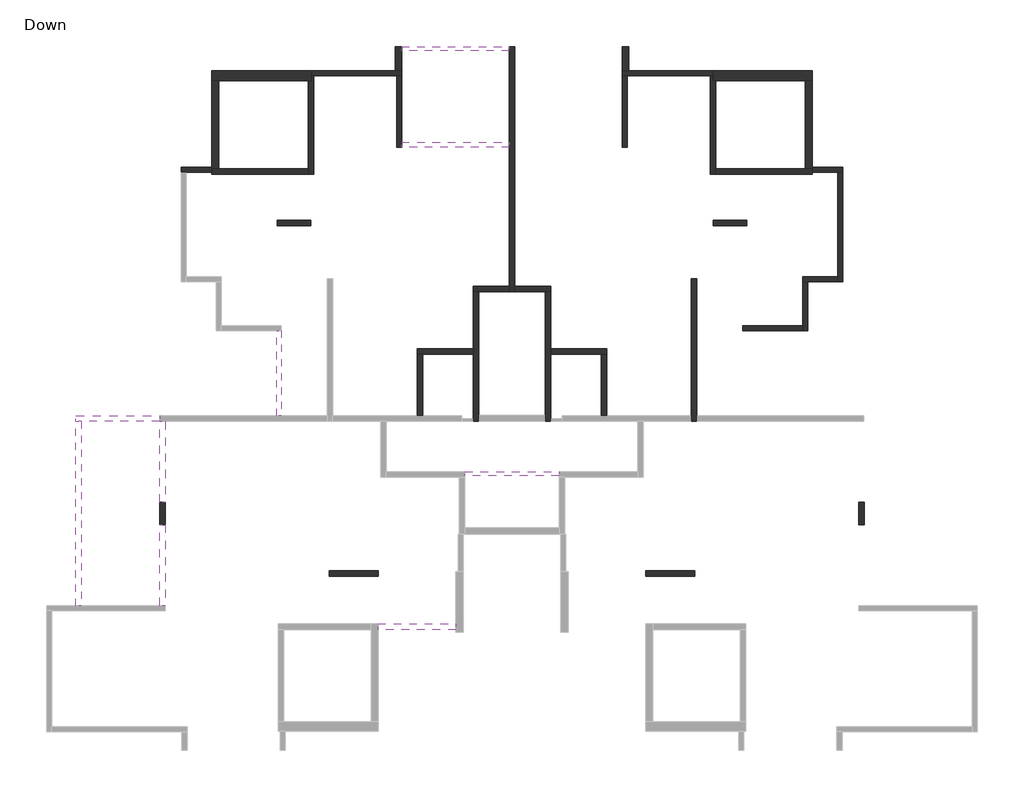
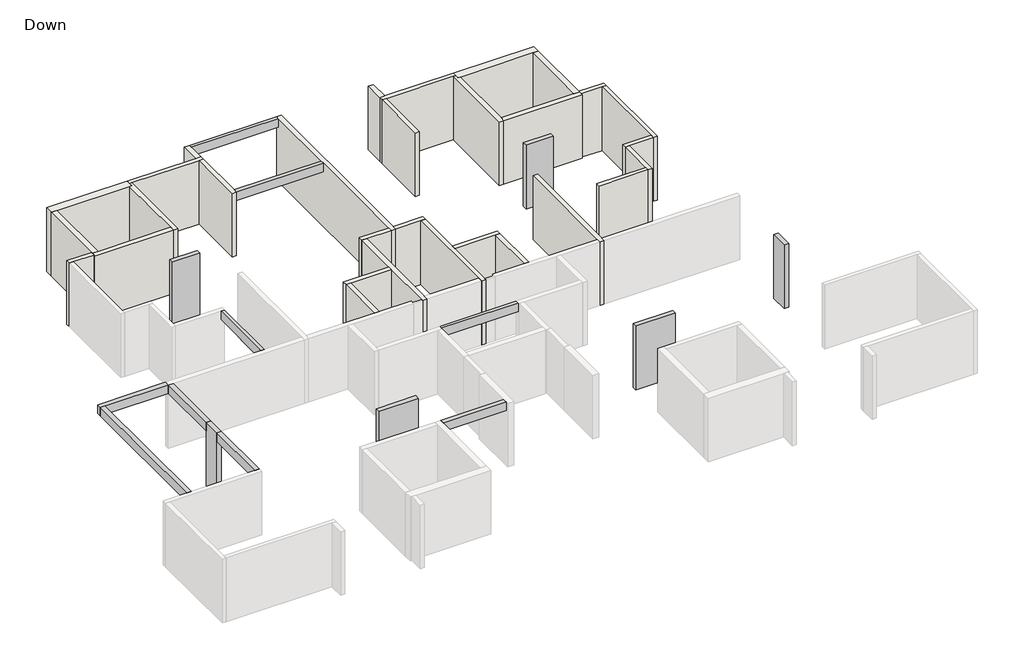
# One storey, part 2 of 2: 30 walls, 9 beams, 6 columns.
"""IFC4 building model written with IfcOpenShell, lengths in millimetres."""

from ifc_helpers import new_model, si_unit, origin, origin_with_axes, place, context, project, spatial, polyline, outline, extrude, faceted_brep, element, save

model = new_model("IFC4")

# Units and contexts
model_context = context("Model", 3, world=origin())
ifc_project = project(units=[si_unit("LENGTHUNIT", "METRE", prefix="MILLI")], contexts=[model_context])

# Site, building, storey
site = spatial("IfcSite", under=ifc_project)
building = spatial("IfcBuilding", under=site)
storey = spatial("IfcBuildingStorey", under=building, Name="Down", Elevation=0.0)

# Beams
placement = place(None, origin())
element("IfcBeam", 1, ObjectType="Concrete Rectengular Beam : 15/40", at=placement, inside=storey, context=model_context, shape_type="Brep", body=[
    faceted_brep([(-7447.2504016, 3105.4959573, 2970.0), (-7597.2504016, 3105.4959573, 2970.0), (-7597.2504016, 53.6346435, 2970.0), (-7447.2504016, 53.6346435, 2970.0), (-7597.2504016, 3105.4959573, 2570.0), (-7597.2504016, 53.6346435, 2570.0), (-7447.2504016, 3105.4959573, 2570.0), (-7447.2504016, 53.6346435, 2570.0), (-7447.2504016, 53.6346435, 2760.0), (-7447.2504016, 3105.4959573, 2760.0)], [[[0, 1, 2, 3]], [[1, 4, 5, 2]], [[4, 6, 7, 5]], [[0, 3, 8, 7, 6, 9]], [[1, 0, 9, 6, 4]], [[3, 2, 5, 7, 8]]]),
])
element("IfcBeam", 2, ObjectType="Concrete Rectengular Beam : 15/40", at=placement, inside=storey, context=model_context, shape_type="Brep", body=[
    faceted_brep([(-3124.7686498, 13277.6127456, 2970.0), (-3124.7686498, 13127.6127456, 2970.0), (722.5306203, 13127.6127456, 2970.0), (722.5306203, 13277.6127456, 2970.0), (-3124.7686498, 13127.6127456, 2760.0), (-3124.7686498, 13127.6127456, 2570.0), (722.5306203, 13127.6127456, 2570.0), (722.5306203, 13127.6127456, 2760.0), (-3124.7686498, 13277.6127456, 2570.0), (722.5306203, 13277.6127456, 2570.0)], [[[0, 1, 2, 3]], [[1, 4, 5, 6, 7, 2]], [[5, 8, 9, 6]], [[8, 0, 3, 9]], [[1, 0, 8, 5, 4]], [[3, 2, 7, 6, 9]]]),
])
element("IfcBeam", 3, ObjectType="Concrete Rectengular Beam : 15/40", at=placement, inside=storey, context=model_context, shape_type="Brep", body=[
    faceted_brep([(-874.5073169, -1946.3653565, 2970.0), (-874.5073169, -2096.3653565, 2970.0), (2519.5685574, -2096.3653565, 2970.0), (2519.5685574, -1946.3653565, 2970.0), (-874.5073169, -2096.3653565, 2760.0), (-874.5073169, -2096.3653565, 2570.0), (2519.5685574, -2096.3653565, 2570.0), (2519.5685574, -2096.3653565, 2760.0), (-874.5073169, -1946.3653565, 2570.0), (2519.5685574, -1946.3653565, 2570.0)], [[[0, 1, 2, 3]], [[1, 4, 5, 6, 7, 2]], [[5, 8, 9, 6]], [[8, 0, 3, 9]], [[1, 0, 8, 5, 4]], [[3, 2, 7, 6, 9]]]),
])
element("IfcBeam", 4, ObjectType="Concrete Rectengular Beam : 18/40", at=placement, inside=storey, context=model_context, shape_type="Brep", body=[
    faceted_brep([(-3124.7686498, 9859.0725997, 2970.0), (-3124.7686498, 9679.0725997, 2970.0), (722.5306203, 9679.0725997, 2970.0), (722.5306203, 9859.0725997, 2970.0), (-3124.7686498, 9679.0725997, 2760.0), (-3124.7686498, 9679.0725997, 2570.0), (722.5306203, 9679.0725997, 2570.0), (722.5306203, 9679.0725997, 2760.0), (-3124.7686498, 9859.0725997, 2570.0), (722.5306203, 9859.0725997, 2570.0), (-3124.7686498, 9859.0725997, 2760.0), (722.5306203, 9859.0725997, 2760.0)], [[[0, 1, 2, 3]], [[2, 1, 4, 5, 6, 7]], [[5, 8, 9, 6]], [[8, 10, 0, 3, 11, 9]], [[1, 0, 10, 8, 5, 4]], [[3, 2, 7, 6, 9, 11]]]),
])
element("IfcBeam", 5, ObjectType="Concrete Rectengular Beam : 20/40", at=placement, inside=storey, context=model_context, shape_type="Brep", body=[
    faceted_brep([(-14797.7613505, 53.6346435, 2970.0), (-14797.7613505, -146.3653565, 2970.0), (-14597.7613505, -146.3653565, 2970.0), (-11795.1336133, -146.3653565, 2970.0), (-11795.1336133, 53.6346435, 2970.0), (-14797.7613505, 53.6346435, 2570.0), (-11795.1336133, 53.6346435, 2570.0), (-14797.7613505, -146.3653565, 2570.0), (-11795.1336133, -146.3653565, 2570.0), (-14597.7613505, -146.3653565, 2570.0), (-11795.1336133, -146.3653565, 2760.0)], [[[0, 1, 2, 3, 4]], [[5, 0, 4, 6]], [[7, 5, 6, 8, 9]], [[1, 7, 9, 8, 10, 3, 2]], [[1, 0, 5, 7]], [[4, 3, 10, 8, 6]]]),
])
element("IfcBeam", 6, ObjectType="Concrete Rectengular Beam : 20/40", at=placement, inside=storey, context=model_context, shape_type="Brep", body=[
    faceted_brep([(-14797.7613505, -6750.8420555, 2970.0), (-14597.7613505, -6750.8420555, 2970.0), (-14597.7613505, -146.3653565, 2970.0), (-14797.7613505, -146.3653565, 2970.0), (-14797.7613505, -6750.8420555, 2570.0), (-14797.7613505, -146.3653565, 2570.0), (-14597.7613505, -6750.8420555, 2570.0), (-14597.7613505, -146.3653565, 2570.0), (-14597.7613505, -6750.8420555, 2760.0), (-14597.7613505, -146.3653565, 2760.0)], [[[0, 1, 2, 3]], [[4, 0, 3, 5]], [[6, 4, 5, 7]], [[1, 8, 6, 7, 9, 2]], [[1, 0, 4, 6, 8]], [[3, 2, 9, 7, 5]]]),
])
element("IfcBeam", 7, ObjectType="Concrete Rectengular Beam : 20/40", at=placement, inside=storey, context=model_context, shape_type="Brep", body=[
    faceted_brep([(-11795.1336133, -3042.8252106, 2970.0), (-11595.1336133, -3042.8252106, 2970.0), (-11595.1336133, -146.3653565, 2970.0), (-11795.1336133, -146.3653565, 2970.0), (-11795.1336133, -3042.8252106, 2570.0), (-11795.1336133, -146.3653565, 2760.0), (-11795.1336133, -146.3653565, 2570.0), (-11595.1336133, -3042.8252106, 2570.0), (-11595.1336133, -146.3653565, 2570.0), (-11595.1336133, -3042.8252106, 2760.0), (-11595.1336133, -146.3653565, 2760.0)], [[[0, 1, 2, 3]], [[4, 0, 3, 5, 6]], [[7, 4, 6, 8]], [[2, 1, 9, 7, 8, 10]], [[1, 0, 4, 7, 9]], [[3, 2, 10, 8, 6, 5]]]),
])
element("IfcBeam", 8, ObjectType="Concrete Rectengular Beam : 20/40", at=placement, inside=storey, context=model_context, shape_type="Brep", body=[
    faceted_brep([(-11595.1336133, -3842.8252106, 2970.0), (-11795.1336133, -3842.8252106, 2970.0), (-11795.1336133, -6750.8420555, 2970.0), (-11595.1336133, -6750.8420555, 2970.0), (-11795.1336133, -3842.8252106, 2570.0), (-11795.1336133, -6750.8420555, 2570.0), (-11795.1336133, -6750.8420555, 2760.0), (-11595.1336133, -3842.8252106, 2570.0), (-11595.1336133, -6750.8420555, 2570.0), (-11595.1336133, -6750.8420555, 2760.0), (-11595.1336133, -3842.8252106, 2760.0)], [[[0, 1, 2, 3]], [[1, 4, 5, 6, 2]], [[4, 7, 8, 5]], [[0, 3, 9, 8, 7, 10]], [[1, 0, 10, 7, 4]], [[3, 2, 6, 5, 8, 9]]]),
])
element("IfcBeam", 9, ObjectType="Concrete Rectengular Beam : 20/40", at=placement, inside=storey, context=model_context, shape_type="Brep", body=[
    faceted_brep([(-3973.7230475, -7395.8420555, 2970.0), (-3973.7230475, -7595.8420555, 2970.0), (-1189.5073169, -7595.8420555, 2970.0), (-1189.5073169, -7395.8420555, 2970.0), (-3973.7230475, -7595.8420555, 2570.0), (-1189.5073169, -7595.8420555, 2570.0), (-3973.7230475, -7395.8420555, 2570.0), (-1189.5073169, -7395.8420555, 2570.0), (-1189.5073169, -7395.8420555, 2760.0), (-3973.7230475, -7395.8420555, 2760.0)], [[[0, 1, 2, 3]], [[1, 4, 5, 2]], [[4, 6, 7, 5]], [[0, 3, 8, 7, 6, 9]], [[1, 0, 9, 6, 4]], [[3, 2, 5, 7, 8]]]),
])

# Columns
element("IfcColumn", 10, ObjectType="Concrete Rectengular Column : 20/120", at=placement, inside=storey, context=model_context, shape_type="Brep", body=[
    faceted_brep([(-7578.4912775, 7053.4886581, 0.0), (-6378.4912775, 7053.4886581, 0.0), (-6378.4912775, 6853.4886581, 0.0), (-7578.4912775, 6853.4886581, 0.0), (-7578.4912775, 7053.4886581, 2970.0), (-6378.4912775, 7053.4886581, 2970.0), (-6378.4912775, 7053.4886581, 2760.0), (-7578.4912775, 7053.4886581, 2760.0), (-6378.4912775, 6853.4886581, 2970.0), (-6378.4912775, 6853.4886581, 2760.0), (-7578.4912775, 6853.4886581, 2970.0), (-7578.4912775, 6853.4886581, 2760.0)], [[[0, 1, 2, 3]], [[4, 5, 6, 1, 0, 7]], [[5, 8, 9, 2, 1, 6]], [[8, 10, 11, 3, 2, 9]], [[10, 4, 7, 0, 3, 11]], [[4, 10, 8, 5]]]),
])
element("IfcColumn", 11, ObjectType="Concrete Rectengular Column : 20/120", at=placement, inside=storey, context=model_context, shape_type="Brep", body=[
    faceted_brep([(9223.5525181, 7053.4886581, 0.0), (9223.5525181, 6853.4886581, 0.0), (8023.5525181, 6853.4886581, 0.0), (8023.5525181, 7053.4886581, 0.0), (9223.5525181, 7053.4886581, 2970.0), (9223.5525181, 7053.4886581, 2760.0), (8023.5525181, 7053.4886581, 2760.0), (8023.5525181, 7053.4886581, 2970.0), (8023.5525181, 6853.4886581, 2760.0), (8023.5525181, 6853.4886581, 2970.0), (9223.5525181, 6853.4886581, 2760.0), (9223.5525181, 6853.4886581, 2970.0)], [[[0, 1, 2, 3]], [[4, 5, 0, 3, 6, 7]], [[7, 6, 3, 2, 8, 9]], [[9, 8, 2, 1, 10, 11]], [[11, 10, 1, 0, 5, 4]], [[4, 7, 9, 11]]]),
])
element("IfcColumn", 12, ObjectType="Concrete Rectengular Column : 20/175", at=placement, inside=storey, context=model_context, shape_type="Brep", body=[
    faceted_brep([(-5724.5402832, -5492.9594837, 0.0), (-3974.5402832, -5492.9594837, 0.0), (-3974.5402832, -5692.9594837, 0.0), (-5724.5402832, -5692.9594837, 0.0), (-5724.5402832, -5492.9594837, 2970.0), (-3974.5402832, -5492.9594837, 2970.0), (-3974.5402832, -5492.9594837, 2760.0), (-5724.5402832, -5492.9594837, 2760.0), (-3974.5402832, -5692.9594837, 2970.0), (-3974.5402832, -5692.9594837, 2760.0), (-5724.5402832, -5692.9594837, 2970.0), (-5724.5402832, -5692.9594837, 2760.0)], [[[0, 1, 2, 3]], [[4, 5, 6, 1, 0, 7]], [[5, 8, 9, 2, 1, 6]], [[8, 10, 11, 3, 2, 9]], [[10, 4, 7, 0, 3, 11]], [[4, 10, 8, 5]]]),
])
element("IfcColumn", 13, ObjectType="Concrete Rectengular Column : 20/175", at=placement, inside=storey, context=model_context, shape_type="Brep", body=[
    faceted_brep([(7369.6015237, -5492.9594837, 0.0), (7369.6015237, -5692.9594837, 0.0), (5619.6015237, -5692.9594837, 0.0), (5619.6015237, -5492.9594837, 0.0), (7369.6015237, -5492.9594837, 2970.0), (7369.6015237, -5492.9594837, 2760.0), (5619.6015237, -5492.9594837, 2760.0), (5619.6015237, -5492.9594837, 2970.0), (5619.6015237, -5692.9594837, 2760.0), (5619.6015237, -5692.9594837, 2970.0), (7369.6015237, -5692.9594837, 2760.0), (7369.6015237, -5692.9594837, 2970.0)], [[[0, 1, 2, 3]], [[4, 5, 0, 3, 6, 7]], [[7, 6, 3, 2, 8, 9]], [[9, 8, 2, 1, 10, 11]], [[11, 10, 1, 0, 5, 4]], [[4, 7, 9, 11]]]),
])
element("IfcColumn", 14, ObjectType="Concrete Rectengular Column : 20/80", at=placement, inside=storey, context=model_context, shape_type="SweptSolid", body=[
    extrude(outline(polyline([(-11595.1336133, -3042.8252106), (-11595.1336133, -3842.8252106), (-11795.1336133, -3842.8252106), (-11795.1336133, -3042.8252106), (-11595.1336133, -3042.8252106)])), origin_with_axes(), (0.0, 0.0, 1.0), 2970.0),
])
element("IfcColumn", 15, ObjectType="Concrete Rectengular Column : 20/80", at=placement, inside=storey, context=model_context, shape_type="SweptSolid", body=[
    extrude(outline(polyline([(13240.1948538, -3042.8252106), (13440.1948538, -3042.8252106), (13440.1948538, -3842.8252106), (13240.1948538, -3842.8252106), (13240.1948538, -3042.8252106)])), origin_with_axes(), (0.0, 0.0, 1.0), 2970.0),
])

# Walls
element("IfcWall", 16, ObjectType="18", at=placement, inside=storey, context=model_context, shape_type="Brep", body=[
    faceted_brep([(-6373.126314, 12225.4959573, 0.0), (-6273.126314, 12225.4959573, 0.0), (-3304.7686498, 12225.4959573, 0.0), (-3124.7686498, 12225.4959573, 0.0), (-3124.7686498, 12225.4959573, 2970.0), (-3304.7686498, 12225.4959573, 2970.0), (-6273.126314, 12225.4959573, 2970.0), (-6373.126314, 12225.4959573, 2970.0), (-6373.126314, 12405.4959573, 0.0), (-6373.126314, 12405.4959573, 2970.0), (-3354.7686498, 12405.4959573, 2970.0), (-3124.7686498, 12405.4959573, 2970.0), (-3124.7686498, 12405.4959573, 0.0), (-3354.7686498, 12405.4959573, 0.0)], [[[0, 1, 2, 3, 4, 5, 6, 7]], [[8, 9, 10, 11, 12, 13]], [[3, 2, 1, 0, 8, 13, 12]], [[7, 6, 5, 4, 11, 10, 9]], [[0, 7, 9, 8]], [[4, 3, 12, 11]]]),
])
element("IfcWall", 17, ObjectType="18", at=placement, inside=storey, context=model_context, shape_type="Brep", body=[
    faceted_brep([(-3304.7686498, 12225.4959573, 0.0), (-3304.7686498, 9679.0725997, 0.0), (-3304.7686498, 9679.0725997, 2760.0), (-3304.7686498, 9679.0725997, 2970.0), (-3304.7686498, 12225.4959573, 2970.0), (-3304.7686498, 12225.4959573, 2760.0), (-3124.7686498, 12225.4959573, 0.0), (-3124.7686498, 12225.4959573, 2970.0), (-3124.7686498, 9859.0725997, 2970.0), (-3124.7686498, 9679.0725997, 2970.0), (-3124.7686498, 9679.0725997, 0.0)], [[[0, 1, 2, 3, 4, 5]], [[6, 7, 8, 9, 10]], [[1, 0, 6, 10]], [[3, 2, 1, 10, 9]], [[4, 3, 9, 8, 7]], [[0, 5, 4, 7, 6]]]),
])
element("IfcWall", 18, ObjectType="18", at=placement, inside=storey, context=model_context, shape_type="Brep", body=[
    faceted_brep([(-9928.126314, 8955.4959573, 0.0), (-11023.126314, 8955.4959573, 0.0), (-11023.126314, 8955.4959573, 2970.0), (-9928.126314, 8955.4959573, 2970.0), (-9928.126314, 8775.4959573, 0.0), (-9928.126314, 8775.4959573, 2760.0), (-9928.126314, 8775.4959573, 2970.0), (-10843.126314, 8775.4959573, 2970.0), (-11023.126314, 8775.4959573, 2970.0), (-11023.126314, 8775.4959573, 0.0), (-10843.126314, 8775.4959573, 0.0), (-9928.126314, 8905.4959573, 0.0), (-9928.126314, 8905.4959573, 2970.0)], [[[0, 1, 2, 3]], [[4, 5, 6, 7, 8, 9, 10]], [[1, 0, 11, 4, 10, 9]], [[3, 2, 8, 7, 6, 12]], [[0, 3, 12, 6, 5, 4, 11]], [[2, 1, 9, 8]]]),
])
element("IfcWall", 19, ObjectType="18", at=placement, inside=storey, context=model_context, shape_type="Brep", body=[
    faceted_brep([(8018.1875546, 12405.4959573, 0.0), (4999.8298903, 12405.4959573, 0.0), (4769.8298903, 12405.4959573, 0.0), (4769.8298903, 12405.4959573, 2970.0), (4999.8298903, 12405.4959573, 2970.0), (8018.1875546, 12405.4959573, 2970.0), (8018.1875546, 12225.4959573, 0.0), (8018.1875546, 12225.4959573, 2970.0), (7918.1875546, 12225.4959573, 2970.0), (4949.8298903, 12225.4959573, 2970.0), (4769.8298903, 12225.4959573, 2970.0), (4769.8298903, 12225.4959573, 0.0), (4949.8298903, 12225.4959573, 0.0), (7918.1875546, 12225.4959573, 0.0)], [[[0, 1, 2, 3, 4, 5]], [[6, 7, 8, 9, 10, 11, 12, 13]], [[2, 1, 0, 6, 13, 12, 11]], [[5, 4, 3, 10, 9, 8, 7]], [[0, 5, 7, 6]], [[3, 2, 11, 10]]]),
])
element("IfcWall", 20, ObjectType="18", at=placement, inside=storey, context=model_context, shape_type="Brep", body=[
    faceted_brep([(4769.8298903, 12225.4959573, 0.0), (4769.8298903, 9679.0725997, 0.0), (4769.8298903, 9679.0725997, 2570.0), (4769.8298903, 9679.0725997, 2970.0), (4769.8298903, 9859.0725997, 2970.0), (4769.8298903, 12225.4959573, 2970.0), (4949.8298903, 12225.4959573, 0.0), (4949.8298903, 12225.4959573, 2760.0), (4949.8298903, 12225.4959573, 2970.0), (4949.8298903, 9679.0725997, 2970.0), (4949.8298903, 9679.0725997, 2760.0), (4949.8298903, 9679.0725997, 0.0)], [[[0, 1, 2, 3, 4, 5]], [[6, 7, 8, 9, 10, 11]], [[1, 0, 6, 11]], [[3, 2, 1, 11, 10, 9]], [[5, 4, 3, 9, 8]], [[0, 5, 8, 7, 6]]]),
])
element("IfcWall", 21, ObjectType="18", at=placement, inside=storey, context=model_context, shape_type="Brep", body=[
    faceted_brep([(11573.1875546, 8775.4959573, 0.0), (12488.1875546, 8775.4959573, 0.0), (12668.1875546, 8775.4959573, 0.0), (12668.1875546, 8775.4959573, 2970.0), (12488.1875546, 8775.4959573, 2970.0), (11573.1875546, 8775.4959573, 2970.0), (11573.1875546, 8775.4959573, 2760.0), (11573.1875546, 8955.4959573, 0.0), (11573.1875546, 8955.4959573, 2970.0), (12668.1875546, 8955.4959573, 2970.0), (12668.1875546, 8955.4959573, 0.0), (11573.1875546, 8905.4959573, 0.0), (11573.1875546, 8905.4959573, 2970.0)], [[[0, 1, 2, 3, 4, 5, 6]], [[7, 8, 9, 10]], [[2, 1, 0, 11, 7, 10]], [[5, 4, 3, 9, 8, 12]], [[0, 6, 5, 12, 8, 7, 11]], [[3, 2, 10, 9]]]),
])
element("IfcWall", 22, ObjectType="18", at=placement, inside=storey, context=model_context, shape_type="Brep", body=[
    faceted_brep([(12488.1875546, 8775.4959573, 0.0), (12488.1875546, 5035.4959573, 0.0), (12488.1875546, 4855.4959573, 0.0), (12488.1875546, 4855.4959573, 2970.0), (12488.1875546, 5035.4959573, 2970.0), (12488.1875546, 8775.4959573, 2970.0), (12488.1875546, 8775.4959573, 2760.0), (12668.1875546, 8775.4959573, 0.0), (12668.1875546, 8775.4959573, 2970.0), (12668.1875546, 4855.4959573, 2970.0), (12668.1875546, 4855.4959573, 0.0)], [[[0, 1, 2, 3, 4, 5, 6]], [[7, 8, 9, 10]], [[2, 1, 0, 7, 10]], [[5, 4, 3, 9, 8]], [[0, 6, 5, 8, 7]], [[3, 2, 10, 9]]]),
])
element("IfcWall", 23, ObjectType="18", at=placement, inside=storey, context=model_context, shape_type="Brep", body=[
    faceted_brep([(12488.1875546, 5035.4959573, 0.0), (11240.6852706, 5035.4959573, 0.0), (11240.6852706, 5035.4959573, 2760.0), (11240.6852706, 5035.4959573, 2970.0), (12488.1875546, 5035.4959573, 2970.0), (12488.1875546, 5035.4959573, 2760.0), (12488.1875546, 4855.4959573, 0.0), (12488.1875546, 4855.4959573, 2970.0), (11420.6852706, 4855.4959573, 2970.0), (11240.6852706, 4855.4959573, 2970.0), (11240.6852706, 4855.4959573, 0.0), (11420.6852706, 4855.4959573, 0.0)], [[[0, 1, 2, 3, 4, 5]], [[6, 7, 8, 9, 10, 11]], [[1, 0, 6, 11, 10]], [[4, 3, 9, 8, 7]], [[0, 5, 4, 7, 6]], [[3, 2, 1, 10, 9]]]),
])
element("IfcWall", 24, ObjectType="18", at=placement, inside=storey, context=model_context, shape_type="Brep", body=[
    faceted_brep([(11240.6852706, 4855.4959573, 0.0), (11240.6852706, 3285.4959573, 0.0), (11240.6852706, 3105.4959573, 0.0), (11240.6852706, 3105.4959573, 2970.0), (11240.6852706, 3285.4959573, 2970.0), (11240.6852706, 4855.4959573, 2970.0), (11420.6852706, 4855.4959573, 0.0), (11420.6852706, 4855.4959573, 2970.0), (11420.6852706, 3105.4959573, 2970.0), (11420.6852706, 3105.4959573, 0.0)], [[[0, 1, 2, 3, 4, 5]], [[6, 7, 8, 9]], [[2, 1, 0, 6, 9]], [[5, 4, 3, 8, 7]], [[0, 5, 7, 6]], [[3, 2, 9, 8]]]),
])
element("IfcWall", 25, ObjectType="18", at=placement, inside=storey, context=model_context, shape_type="Brep", body=[
    faceted_brep([(11240.6852706, 3285.4959573, 0.0), (9090.6852706, 3285.4959573, 0.0), (9090.6852706, 3285.4959573, 2760.0), (9090.6852706, 3285.4959573, 2970.0), (11240.6852706, 3285.4959573, 2970.0), (11240.6852706, 3285.4959573, 2760.0), (11240.6852706, 3105.4959573, 0.0), (11240.6852706, 3105.4959573, 2970.0), (9092.3116422, 3105.4959573, 2970.0), (9090.6852706, 3105.4959573, 2970.0), (9090.6852706, 3105.4959573, 2760.0), (9090.6852706, 3105.4959573, 0.0)], [[[0, 1, 2, 3, 4, 5]], [[6, 7, 8, 9, 10, 11]], [[1, 0, 6, 11]], [[3, 2, 1, 11, 10, 9]], [[4, 3, 9, 8, 7]], [[0, 5, 4, 7, 6]]]),
])
element("IfcWall", 26, ObjectType="20", at=placement, inside=storey, context=model_context, shape_type="Brep", body=[
    faceted_brep([(-6473.126314, 12055.4959573, 0.0), (-6473.126314, 8905.4959573, 0.0), (-6473.126314, 8705.4959573, 0.0), (-6473.126314, 8705.4959573, 2970.0), (-6473.126314, 8905.4959573, 2970.0), (-6473.126314, 12055.4959573, 2970.0), (-6473.126314, 12055.4959573, 2760.0), (-6273.126314, 12225.4959573, 0.0), (-6273.126314, 12225.4959573, 2760.0), (-6273.126314, 12225.4959573, 2970.0), (-6273.126314, 8705.4959573, 2970.0), (-6273.126314, 8705.4959573, 2760.0), (-6273.126314, 8705.4959573, 0.0), (-6373.126314, 12055.4959573, 0.0), (-6373.126314, 12225.4959573, 0.0), (-6373.126314, 12225.4959573, 2970.0), (-6373.126314, 12055.4959573, 2970.0)], [[[0, 1, 2, 3, 4, 5, 6]], [[7, 8, 9, 10, 11, 12]], [[2, 1, 0, 13, 14, 7, 12]], [[5, 4, 3, 10, 9, 15, 16]], [[0, 6, 5, 16, 13]], [[16, 15, 14, 13]], [[15, 9, 8, 7, 14]], [[3, 2, 12, 11, 10]]]),
])
element("IfcWall", 27, ObjectType="20", at=placement, inside=storey, context=model_context, shape_type="Brep", body=[
    faceted_brep([(-6473.126314, 8905.4959573, 0.0), (-9678.126314, 8905.4959573, 0.0), (-9928.126314, 8905.4959573, 0.0), (-9928.126314, 8905.4959573, 2970.0), (-9678.126314, 8905.4959573, 2970.0), (-6473.126314, 8905.4959573, 2970.0), (-6473.126314, 8905.4959573, 2760.0), (-6473.126314, 8705.4959573, 0.0), (-6473.126314, 8705.4959573, 2970.0), (-9928.126314, 8705.4959573, 2970.0), (-9928.126314, 8705.4959573, 2760.0), (-9928.126314, 8705.4959573, 0.0), (-9928.126314, 8775.4959573, 0.0), (-9928.126314, 8775.4959573, 2970.0)], [[[0, 1, 2, 3, 4, 5, 6]], [[7, 8, 9, 10, 11]], [[2, 1, 0, 7, 11, 12]], [[5, 4, 3, 13, 9, 8]], [[0, 6, 5, 8, 7]], [[3, 2, 12, 11, 10, 9, 13]]]),
])
element("IfcWall", 28, ObjectType="20", at=placement, inside=storey, context=model_context, shape_type="Brep", body=[
    faceted_brep([(722.5306203, 13277.6127456, 0.0), (722.5306203, 4702.6127456, 0.0), (722.5306203, 4502.6127456, 0.0), (722.5306203, 4502.6127456, 2970.0), (722.5306203, 4702.6127456, 2970.0), (722.5306203, 9679.0725997, 2970.0), (722.5306203, 9859.0725997, 2970.0), (722.5306203, 13127.6127456, 2970.0), (722.5306203, 13277.6127456, 2970.0), (922.5306203, 13277.6127456, 0.0), (922.5306203, 13277.6127456, 2970.0), (922.5306203, 13127.6127456, 2970.0), (922.5306203, 9859.0725997, 2970.0), (922.5306203, 9679.0725997, 2970.0), (922.5306203, 4702.6127456, 2970.0), (922.5306203, 4502.6127456, 2970.0), (922.5306203, 4502.6127456, 0.0), (922.5306203, 4702.6127456, 0.0)], [[[0, 1, 2, 3, 4, 5, 6, 7, 8]], [[9, 10, 11, 12, 13, 14, 15, 16, 17]], [[2, 1, 0, 9, 17, 16]], [[8, 7, 6, 5, 4, 3, 15, 14, 13, 12, 11, 10]], [[0, 8, 10, 9]], [[3, 2, 16, 15]]]),
])
element("IfcWall", 29, ObjectType="20", at=placement, inside=storey, context=model_context, shape_type="Brep", body=[
    faceted_brep([(722.5306203, 4702.6127456, 0.0), (-572.4693797, 4702.6127456, 0.0), (-572.4693797, 4702.6127456, 2760.0), (-572.4693797, 4702.6127456, 2970.0), (722.5306203, 4702.6127456, 2970.0), (722.5306203, 4702.6127456, 2760.0), (722.5306203, 4502.6127456, 0.0), (722.5306203, 4502.6127456, 2970.0), (-372.4693797, 4502.6127456, 2970.0), (-572.4693797, 4502.6127456, 2970.0), (-572.4693797, 4502.6127456, 0.0), (-372.4693797, 4502.6127456, 0.0)], [[[0, 1, 2, 3, 4, 5]], [[6, 7, 8, 9, 10, 11]], [[1, 0, 6, 11, 10]], [[4, 3, 9, 8, 7]], [[0, 5, 4, 7, 6]], [[3, 2, 1, 10, 9]]]),
])
element("IfcWall", 30, ObjectType="20", at=placement, inside=storey, context=model_context, shape_type="Brep", body=[
    faceted_brep([(-572.4693797, 4502.6127456, 0.0), (-572.4693797, 2452.6127456, 0.0), (-572.4693797, 2252.6127456, 0.0), (-572.4693797, -46.3653565, 0.0), (-572.4693797, -146.3653565, 0.0), (-572.4693797, -146.3653565, 2970.0), (-572.4693797, -46.3653565, 2970.0), (-572.4693797, 2252.6127456, 2970.0), (-572.4693797, 2452.6127456, 2970.0), (-572.4693797, 4502.6127456, 2970.0), (-372.4693797, 4502.6127456, 0.0), (-372.4693797, 4502.6127456, 2970.0), (-372.4693797, 83.6346435, 2970.0), (-372.4693797, -146.3653565, 2970.0), (-372.4693797, -146.3653565, 0.0), (-372.4693797, 83.6346435, 0.0)], [[[0, 1, 2, 3, 4, 5, 6, 7, 8, 9]], [[10, 11, 12, 13, 14, 15]], [[4, 3, 2, 1, 0, 10, 15, 14]], [[9, 8, 7, 6, 5, 13, 12, 11]], [[0, 9, 11, 10]], [[5, 4, 14, 13]]]),
])
element("IfcWall", 31, ObjectType="20", at=placement, inside=storey, context=model_context, shape_type="Brep", body=[
    faceted_brep([(-572.4693797, 2452.6127456, 0.0), (-2572.4693797, 2452.6127456, 0.0), (-2572.4693797, 2452.6127456, 2760.0), (-2572.4693797, 2452.6127456, 2970.0), (-572.4693797, 2452.6127456, 2970.0), (-572.4693797, 2452.6127456, 2760.0), (-572.4693797, 2252.6127456, 0.0), (-572.4693797, 2252.6127456, 2970.0), (-2372.4693797, 2252.6127456, 2970.0), (-2572.4693797, 2252.6127456, 2970.0), (-2572.4693797, 2252.6127456, 0.0), (-2372.4693797, 2252.6127456, 0.0)], [[[0, 1, 2, 3, 4, 5]], [[6, 7, 8, 9, 10, 11]], [[1, 0, 6, 11, 10]], [[4, 3, 9, 8, 7]], [[0, 5, 4, 7, 6]], [[3, 2, 1, 10, 9]]]),
])
element("IfcWall", 32, ObjectType="20", at=placement, inside=storey, context=model_context, shape_type="Brep", body=[
    faceted_brep([(-2572.4693797, 2252.6127456, 0.0), (-2572.4693797, 53.6346435, 0.0), (-2572.4693797, 53.6346435, 2760.0), (-2572.4693797, 53.6346435, 2970.0), (-2572.4693797, 2252.6127456, 2970.0), (-2372.4693797, 2252.6127456, 0.0), (-2372.4693797, 2252.6127456, 2970.0), (-2372.4693797, 53.6346435, 2970.0), (-2372.4693797, 53.6346435, 0.0)], [[[0, 1, 2, 3, 4]], [[5, 6, 7, 8]], [[1, 0, 5, 8]], [[4, 3, 7, 6]], [[0, 4, 6, 5]], [[3, 2, 1, 8, 7]]]),
])
element("IfcWall", 33, ObjectType="20", at=placement, inside=storey, context=model_context, shape_type="Brep", body=[
    faceted_brep([(7918.1875546, 12225.4959573, 0.0), (7918.1875546, 8705.4959573, 0.0), (7918.1875546, 8705.4959573, 2760.0), (7918.1875546, 8705.4959573, 2970.0), (7918.1875546, 12225.4959573, 2970.0), (7918.1875546, 12225.4959573, 2760.0), (8118.1875546, 12055.4959573, 0.0), (8118.1875546, 12055.4959573, 2760.0), (8118.1875546, 12055.4959573, 2970.0), (8118.1875546, 8905.4959573, 2970.0), (8118.1875546, 8705.4959573, 2970.0), (8118.1875546, 8705.4959573, 0.0), (8118.1875546, 8905.4959573, 0.0), (8018.1875546, 12225.4959573, 0.0), (8018.1875546, 12055.4959573, 0.0), (8018.1875546, 12055.4959573, 2970.0), (8018.1875546, 12225.4959573, 2970.0)], [[[0, 1, 2, 3, 4, 5]], [[6, 7, 8, 9, 10, 11, 12]], [[1, 0, 13, 14, 6, 12, 11]], [[4, 3, 10, 9, 8, 15, 16]], [[0, 5, 4, 16, 13]], [[16, 15, 14, 13]], [[15, 8, 7, 6, 14]], [[3, 2, 1, 11, 10]]]),
])
element("IfcWall", 34, ObjectType="20", at=placement, inside=storey, context=model_context, shape_type="Brep", body=[
    faceted_brep([(8118.1875546, 8705.4959573, 0.0), (11573.1875546, 8705.4959573, 0.0), (11573.1875546, 8705.4959573, 2760.0), (11573.1875546, 8705.4959573, 2970.0), (8118.1875546, 8705.4959573, 2970.0), (8118.1875546, 8905.4959573, 0.0), (8118.1875546, 8905.4959573, 2760.0), (8118.1875546, 8905.4959573, 2970.0), (11323.1875546, 8905.4959573, 2970.0), (11573.1875546, 8905.4959573, 2970.0), (11573.1875546, 8905.4959573, 0.0), (11323.1875546, 8905.4959573, 0.0), (11573.1875546, 8775.4959573, 0.0), (11573.1875546, 8775.4959573, 2970.0)], [[[0, 1, 2, 3, 4]], [[5, 6, 7, 8, 9, 10, 11]], [[1, 0, 5, 11, 10, 12]], [[4, 3, 13, 9, 8, 7]], [[0, 4, 7, 6, 5]], [[3, 2, 1, 12, 10, 9, 13]]]),
])
element("IfcWall", 35, ObjectType="20", at=placement, inside=storey, context=model_context, shape_type="Brep", body=[
    faceted_brep([(7242.2386495, 4958.6346435, 0.0), (7242.2386495, 53.6346435, 0.0), (7242.2386495, -146.3653565, 0.0), (7242.2386495, -146.3653565, 2970.0), (7242.2386495, 53.6346435, 2970.0), (7242.2386495, 4958.6346435, 2970.0), (7242.2386495, 4958.6346435, 2760.0), (7442.2386495, 4958.6346435, 0.0), (7442.2386495, 4958.6346435, 2760.0), (7442.2386495, 4958.6346435, 2970.0), (7442.2386495, 53.6346435, 2970.0), (7442.2386495, -146.3653565, 2970.0), (7442.2386495, -146.3653565, 0.0), (7442.2386495, 53.6346435, 0.0)], [[[0, 1, 2, 3, 4, 5, 6]], [[7, 8, 9, 10, 11, 12, 13]], [[2, 1, 0, 7, 13, 12]], [[5, 4, 3, 11, 10, 9]], [[0, 6, 5, 9, 8, 7]], [[3, 2, 12, 11]]]),
])
element("IfcWall", 36, ObjectType="20", at=placement, inside=storey, context=model_context, shape_type="Brep", body=[
    faceted_brep([(922.5306203, 4502.6127456, 0.0), (2017.5306203, 4502.6127456, 0.0), (2217.5306203, 4502.6127456, 0.0), (2217.5306203, 4502.6127456, 2970.0), (2017.5306203, 4502.6127456, 2970.0), (922.5306203, 4502.6127456, 2970.0), (922.5306203, 4702.6127456, 0.0), (922.5306203, 4702.6127456, 2760.0), (922.5306203, 4702.6127456, 2970.0), (2217.5306203, 4702.6127456, 2970.0), (2217.5306203, 4702.6127456, 2760.0), (2217.5306203, 4702.6127456, 0.0)], [[[0, 1, 2, 3, 4, 5]], [[6, 7, 8, 9, 10, 11]], [[2, 1, 0, 6, 11]], [[5, 4, 3, 9, 8]], [[3, 2, 11, 10, 9]], [[0, 5, 8, 7, 6]]]),
])
element("IfcWall", 37, ObjectType="20", at=placement, inside=storey, context=model_context, shape_type="Brep", body=[
    faceted_brep([(2017.5306203, 4502.6127456, 0.0), (2017.5306203, 83.6346435, 0.0), (2017.5306203, -146.3653565, 0.0), (2017.5306203, -146.3653565, 2970.0), (2017.5306203, 83.6346435, 2970.0), (2017.5306203, 4502.6127456, 2970.0), (2217.5306203, 4502.6127456, 0.0), (2217.5306203, 4502.6127456, 2970.0), (2217.5306203, 2452.6127456, 2970.0), (2217.5306203, 2252.6127456, 2970.0), (2217.5306203, -46.3653565, 2970.0), (2217.5306203, -146.3653565, 2970.0), (2217.5306203, -146.3653565, 0.0), (2217.5306203, -46.3653565, 0.0), (2217.5306203, 2252.6127456, 0.0), (2217.5306203, 2452.6127456, 0.0)], [[[0, 1, 2, 3, 4, 5]], [[6, 7, 8, 9, 10, 11, 12, 13, 14, 15]], [[2, 1, 0, 6, 15, 14, 13, 12]], [[5, 4, 3, 11, 10, 9, 8, 7]], [[0, 5, 7, 6]], [[3, 2, 12, 11]]]),
])
element("IfcWall", 38, ObjectType="20", at=placement, inside=storey, context=model_context, shape_type="Brep", body=[
    faceted_brep([(2217.5306203, 2252.6127456, 0.0), (4017.5306203, 2252.6127456, 0.0), (4217.5306203, 2252.6127456, 0.0), (4217.5306203, 2252.6127456, 2970.0), (4017.5306203, 2252.6127456, 2970.0), (2217.5306203, 2252.6127456, 2970.0), (2217.5306203, 2452.6127456, 0.0), (2217.5306203, 2452.6127456, 2760.0), (2217.5306203, 2452.6127456, 2970.0), (4217.5306203, 2452.6127456, 2970.0), (4217.5306203, 2452.6127456, 2760.0), (4217.5306203, 2452.6127456, 0.0)], [[[0, 1, 2, 3, 4, 5]], [[6, 7, 8, 9, 10, 11]], [[2, 1, 0, 6, 11]], [[5, 4, 3, 9, 8]], [[0, 5, 8, 7, 6]], [[3, 2, 11, 10, 9]]]),
])
element("IfcWall", 39, ObjectType="20", at=placement, inside=storey, context=model_context, shape_type="Brep", body=[
    faceted_brep([(4017.5306203, 2252.6127456, 0.0), (4017.5306203, 53.6346435, 0.0), (4017.5306203, 53.6346435, 2970.0), (4017.5306203, 2252.6127456, 2970.0), (4217.5306203, 2252.6127456, 0.0), (4217.5306203, 2252.6127456, 2970.0), (4217.5306203, 53.6346435, 2970.0), (4217.5306203, 53.6346435, 2760.0), (4217.5306203, 53.6346435, 0.0)], [[[0, 1, 2, 3]], [[4, 5, 6, 7, 8]], [[1, 0, 4, 8]], [[3, 2, 6, 5]], [[0, 3, 5, 4]], [[2, 1, 8, 7, 6]]]),
])
element("IfcWall", 40, ObjectType="23", at=placement, inside=storey, context=model_context, shape_type="Brep", body=[
    faceted_brep([(-3124.7686498, 12405.4959573, 0.0), (-3124.7686498, 13277.6127456, 0.0), (-3124.7686498, 13277.6127456, 2970.0), (-3124.7686498, 13127.6127456, 2970.0), (-3124.7686498, 12405.4959573, 2970.0), (-3354.7686498, 12405.4959573, 0.0), (-3354.7686498, 12405.4959573, 2970.0), (-3354.7686498, 13277.6127456, 2970.0), (-3354.7686498, 13277.6127456, 0.0)], [[[0, 1, 2, 3, 4]], [[5, 6, 7, 8]], [[1, 0, 5, 8]], [[2, 1, 8, 7]], [[4, 3, 2, 7, 6]], [[0, 4, 6, 5]]]),
])
element("IfcWall", 41, ObjectType="23", at=placement, inside=storey, context=model_context, shape_type="Brep", body=[
    faceted_brep([(4999.8298903, 12405.4959573, 0.0), (4999.8298903, 13277.6127456, 0.0), (4999.8298903, 13277.6127456, 2970.0), (4999.8298903, 12405.4959573, 2970.0), (4769.8298903, 12405.4959573, 0.0), (4769.8298903, 12405.4959573, 2970.0), (4769.8298903, 13127.6127456, 2970.0), (4769.8298903, 13277.6127456, 2970.0), (4769.8298903, 13277.6127456, 0.0)], [[[0, 1, 2, 3]], [[4, 5, 6, 7, 8]], [[1, 0, 4, 8]], [[2, 1, 8, 7]], [[3, 2, 7, 6, 5]], [[0, 3, 5, 4]]]),
])
element("IfcWall", 42, ObjectType="25", at=placement, inside=storey, context=model_context, shape_type="Brep", body=[
    faceted_brep([(-9928.126314, 12055.4959573, 0.0), (-9928.126314, 8955.4959573, 0.0), (-9928.126314, 8905.4959573, 0.0), (-9928.126314, 8905.4959573, 2970.0), (-9928.126314, 8955.4959573, 2970.0), (-9928.126314, 12055.4959573, 2970.0), (-9678.126314, 12055.4959573, 0.0), (-9678.126314, 12055.4959573, 2760.0), (-9678.126314, 12055.4959573, 2970.0), (-9678.126314, 8905.4959573, 2970.0), (-9678.126314, 8905.4959573, 2760.0), (-9678.126314, 8905.4959573, 0.0)], [[[0, 1, 2, 3, 4, 5]], [[6, 7, 8, 9, 10, 11]], [[2, 1, 0, 6, 11]], [[5, 4, 3, 9, 8]], [[0, 5, 8, 7, 6]], [[3, 2, 11, 10, 9]]]),
])
element("IfcWall", 43, ObjectType="25", at=placement, inside=storey, context=model_context, shape_type="Brep", body=[
    faceted_brep([(11323.1875546, 12055.4959573, 0.0), (11323.1875546, 8905.4959573, 0.0), (11323.1875546, 8905.4959573, 2760.0), (11323.1875546, 8905.4959573, 2970.0), (11323.1875546, 12055.4959573, 2970.0), (11323.1875546, 12055.4959573, 2760.0), (11573.1875546, 12055.4959573, 0.0), (11573.1875546, 12055.4959573, 2970.0), (11573.1875546, 8955.4959573, 2970.0), (11573.1875546, 8905.4959573, 2970.0), (11573.1875546, 8905.4959573, 0.0), (11573.1875546, 8955.4959573, 0.0)], [[[0, 1, 2, 3, 4, 5]], [[6, 7, 8, 9, 10, 11]], [[1, 0, 6, 11, 10]], [[4, 3, 9, 8, 7]], [[0, 5, 4, 7, 6]], [[3, 2, 1, 10, 9]]]),
])
element("IfcWall", 44, ObjectType="35", at=placement, inside=storey, context=model_context, shape_type="Brep", body=[
    faceted_brep([(-9928.126314, 12055.4959573, 0.0), (-9678.126314, 12055.4959573, 0.0), (-6473.126314, 12055.4959573, 0.0), (-6373.126314, 12055.4959573, 0.0), (-6373.126314, 12055.4959573, 2970.0), (-6473.126314, 12055.4959573, 2970.0), (-9678.126314, 12055.4959573, 2970.0), (-9928.126314, 12055.4959573, 2970.0), (-9928.126314, 12405.4959573, 0.0), (-9928.126314, 12405.4959573, 2970.0), (-6373.126314, 12405.4959573, 2970.0), (-6373.126314, 12405.4959573, 0.0), (-6373.126314, 12225.4959573, 0.0), (-6373.126314, 12225.4959573, 2970.0)], [[[0, 1, 2, 3, 4, 5, 6, 7]], [[8, 9, 10, 11]], [[3, 2, 1, 0, 8, 11, 12]], [[4, 3, 12, 11, 10, 13]], [[7, 6, 5, 4, 13, 10, 9]], [[0, 7, 9, 8]]]),
])
element("IfcWall", 45, ObjectType="35", at=placement, inside=storey, context=model_context, shape_type="Brep", body=[
    faceted_brep([(11573.1875546, 12405.4959573, 0.0), (8018.1875546, 12405.4959573, 0.0), (8018.1875546, 12405.4959573, 2970.0), (11573.1875546, 12405.4959573, 2970.0), (11573.1875546, 12055.4959573, 0.0), (11573.1875546, 12055.4959573, 2970.0), (11323.1875546, 12055.4959573, 2970.0), (8118.1875546, 12055.4959573, 2970.0), (8018.1875546, 12055.4959573, 2970.0), (8018.1875546, 12055.4959573, 0.0), (8118.1875546, 12055.4959573, 0.0), (11323.1875546, 12055.4959573, 0.0), (8018.1875546, 12225.4959573, 0.0), (8018.1875546, 12225.4959573, 2970.0)], [[[0, 1, 2, 3]], [[4, 5, 6, 7, 8, 9, 10, 11]], [[1, 0, 4, 11, 10, 9, 12]], [[2, 1, 12, 9, 8, 13]], [[3, 2, 13, 8, 7, 6, 5]], [[0, 3, 5, 4]]]),
])

save(model, "model.ifc")

# Revit data of these elements
# Type "Concrete Rectengular Beam : 15/40"
#   Length [instance default] = 152.4 cm
#   b = 15 cm
#   h = 40 cm
#   Structural Material [instance default] = Concrete
#   Assembly Code = ""
# Type "Concrete Rectengular Beam : 18/40"
#   Length [instance default] = 152.4 cm
#   b = 18 cm
#   h = 40 cm
#   Structural Material [instance default] = Concrete
#   Assembly Code = ""
# Type "Concrete Rectengular Beam : 20/40"
#   Keynote = "09000"
#   Length [instance default] = 152.4 cm
#   b = 20 cm
#   h = 40 cm
#   Structural Material [instance default] = Concrete
#   Assembly Code = ""
# Type "Concrete Rectengular Column : 20/120"
#   b = 20 cm
#   h = 120 cm
#   Structural Material [instance default] = Concrete
# Type "Concrete Rectengular Column : 20/175"
#   b = 20 cm
#   h = 175 cm
#   Structural Material [instance default] = Concrete
# Type "Concrete Rectengular Column : 20/80"
#   b = 20 cm
#   h = 80 cm
#   Structural Material [instance default] = Concrete
# Type "18"
#   Layers, outside or top first: 18 cm "Concrete" (function 1)
# Type "20"
#   Layers, outside or top first: 20 cm "Concrete" (function 1)
# Type "23"
#   Layers, outside or top first: 23 cm "Concrete" (function 1)
# Type "25"
#   Layers, outside or top first: 25 cm "Concrete" (function 1)
# Type "35"
#   Layers, outside or top first: 35 cm "Concrete" (function 1)
# Element 1 (IfcBeam, "Concrete Rectengular Beam : 15/40")
#   Comments = ""
#   Mark = "B1"
#   SOFiSTiK_AMG_Comments = ""
#   SOFiSTiK_AMG_Scheduled = yes
#   SOFiSTiK_AMG_Adjusted = yes
#   Structural Material = Concrete
#   Phase Created = New Construction
#   Materials on its faces: "Concrete"
# Element 2 (IfcBeam, "Concrete Rectengular Beam : 15/40")
#   Comments = ""
#   Mark = "B2"
#   SOFiSTiK_AMG_Comments = ""
#   SOFiSTiK_AMG_Scheduled = yes
#   SOFiSTiK_AMG_Adjusted = yes
#   Structural Material = Concrete
#   Phase Created = New Construction
#   Materials on its faces: "Concrete"
# Element 3 (IfcBeam, "Concrete Rectengular Beam : 15/40")
#   Comments = ""
#   Mark = "B5"
#   SOFiSTiK_AMG_Comments = ""
#   SOFiSTiK_AMG_Scheduled = yes
#   SOFiSTiK_AMG_Adjusted = yes
#   Structural Material = Concrete
#   Phase Created = New Construction
#   Materials on its faces: "Concrete"
# Element 4 (IfcBeam, "Concrete Rectengular Beam : 18/40")
#   Comments = ""
#   Mark = "B6"
#   SOFiSTiK_AMG_Comments = ""
#   SOFiSTiK_AMG_Scheduled = yes
#   SOFiSTiK_AMG_Adjusted = yes
#   Structural Material = Concrete
#   Phase Created = New Construction
#   Materials on its faces: "Concrete"
# Element 5 (IfcBeam, "Concrete Rectengular Beam : 20/40")
#   Comments = ""
#   Mark = "B8"
#   SOFiSTiK_AMG_Comments = ""
#   SOFiSTiK_AMG_Scheduled = yes
#   SOFiSTiK_AMG_Adjusted = yes
#   Structural Material = Concrete
#   Phase Created = New Construction
#   Materials on its faces: "Concrete"
# Element 6 (IfcBeam, "Concrete Rectengular Beam : 20/40")
#   Comments = ""
#   Mark = "B9"
#   SOFiSTiK_AMG_Comments = ""
#   SOFiSTiK_AMG_Scheduled = yes
#   SOFiSTiK_AMG_Adjusted = yes
#   Structural Material = Concrete
#   Phase Created = New Construction
#   Materials on its faces: "Concrete"
# Element 7 (IfcBeam, "Concrete Rectengular Beam : 20/40")
#   Comments = ""
#   Mark = "B10"
#   SOFiSTiK_AMG_Comments = ""
#   SOFiSTiK_AMG_Scheduled = yes
#   SOFiSTiK_AMG_Adjusted = yes
#   Structural Material = Concrete
#   Phase Created = New Construction
#   Materials on its faces: "Concrete"
# Element 8 (IfcBeam, "Concrete Rectengular Beam : 20/40")
#   Comments = ""
#   Mark = "B11"
#   SOFiSTiK_AMG_Comments = ""
#   SOFiSTiK_AMG_Scheduled = yes
#   SOFiSTiK_AMG_Adjusted = yes
#   Structural Material = Concrete
#   Phase Created = New Construction
#   Materials on its faces: "Concrete"
# Element 9 (IfcBeam, "Concrete Rectengular Beam : 20/40")
#   Comments = ""
#   Mark = "B12"
#   SOFiSTiK_AMG_Comments = ""
#   SOFiSTiK_AMG_Scheduled = yes
#   SOFiSTiK_AMG_Adjusted = yes
#   Structural Material = Concrete
#   Phase Created = New Construction
#   Materials on its faces: "Concrete"
# Element 10 (IfcColumn, "Concrete Rectengular Column : 20/120")
#   Comments = ""
#   Mark = "C1"
#   SOFiSTiK_AMG_Comments = ""
#   SOFiSTiK_AMG_Scheduled = yes
#   SOFiSTiK_AMG_Adjusted = yes
#   Structural Material = Concrete
#   Phase Created = New Construction
#   Materials on its faces: "Concrete"
# Element 11 (IfcColumn, "Concrete Rectengular Column : 20/120")
#   Comments = ""
#   Mark = "C2"
#   SOFiSTiK_AMG_Comments = ""
#   SOFiSTiK_AMG_Scheduled = yes
#   SOFiSTiK_AMG_Adjusted = yes
#   Structural Material = Concrete
#   Phase Created = New Construction
#   Materials on its faces: "Concrete"
# Element 12 (IfcColumn, "Concrete Rectengular Column : 20/175")
#   Comments = ""
#   Mark = "C3"
#   SOFiSTiK_AMG_Comments = ""
#   SOFiSTiK_AMG_Scheduled = yes
#   SOFiSTiK_AMG_Adjusted = yes
#   Structural Material = Concrete
#   Phase Created = New Construction
#   Materials on its faces: "Concrete"
# Element 13 (IfcColumn, "Concrete Rectengular Column : 20/175")
#   Comments = ""
#   Mark = "C4"
#   SOFiSTiK_AMG_Comments = ""
#   SOFiSTiK_AMG_Scheduled = yes
#   SOFiSTiK_AMG_Adjusted = yes
#   Structural Material = Concrete
#   Phase Created = New Construction
#   Materials on its faces: "Concrete"
# Element 14 (IfcColumn, "Concrete Rectengular Column : 20/80")
#   Comments = ""
#   Mark = "C5"
#   SOFiSTiK_AMG_Comments = ""
#   SOFiSTiK_AMG_Scheduled = yes
#   SOFiSTiK_AMG_Adjusted = yes
#   Structural Material = Concrete
#   Phase Created = New Construction
#   Materials on its faces: "Concrete"
# Element 15 (IfcColumn, "Concrete Rectengular Column : 20/80")
#   Comments = ""
#   Mark = "C6"
#   SOFiSTiK_AMG_Comments = ""
#   SOFiSTiK_AMG_Scheduled = yes
#   SOFiSTiK_AMG_Adjusted = yes
#   Structural Material = Concrete
#   Phase Created = New Construction
#   Materials on its faces: "Concrete"
# Element 16 (IfcWall, "18")
#   Comments = ""
#   Mark = "W5"
#   SOFiSTiK_EdgeZones = "W5"
#   SOFiSTiK_AMG_Comments = ""
#   Top Offset = 0 cm
#   Base Offset = 0 cm
#   wall height = 297 cm
#   SOFiSTiK_AMG_Scheduled = yes
#   SOFiSTiK_AMG_Adjusted = yes
#   Phase Created = New Construction
#   Base Constraint = Down
#   Top Constraint = Typical Floor
#   Materials on its faces: "Concrete"
# Element 17 (IfcWall, "18")
#   Comments = ""
#   Mark = "W6"
#   SOFiSTiK_EdgeZones = "W6"
#   SOFiSTiK_AMG_Comments = ""
#   Top Offset = 0 cm
#   Base Offset = 0 cm
#   wall height = 297 cm
#   SOFiSTiK_AMG_Scheduled = yes
#   SOFiSTiK_AMG_Adjusted = yes
#   Phase Created = New Construction
#   Base Constraint = Down
#   Top Constraint = Typical Floor
#   Materials on its faces: "Concrete"
# Element 18 (IfcWall, "18")
#   Comments = ""
#   Mark = "W7"
#   SOFiSTiK_EdgeZones = "W7"
#   SOFiSTiK_AMG_Comments = ""
#   Top Offset = 0 cm
#   Base Offset = 0 cm
#   wall height = 297 cm
#   SOFiSTiK_AMG_Scheduled = yes
#   SOFiSTiK_AMG_Adjusted = yes
#   Phase Created = New Construction
#   Base Constraint = Down
#   Top Constraint = Typical Floor
#   Materials on its faces: "Concrete"
# Element 19 (IfcWall, "18")
#   Comments = ""
#   Mark = "W19"
#   SOFiSTiK_EdgeZones = "W19"
#   SOFiSTiK_AMG_Comments = ""
#   Top Offset = 0 cm
#   Base Offset = 0 cm
#   wall height = 297 cm
#   SOFiSTiK_AMG_Scheduled = yes
#   SOFiSTiK_AMG_Adjusted = yes
#   Phase Created = New Construction
#   Base Constraint = Down
#   Top Constraint = Typical Floor
#   Materials on its faces: "Concrete"
# Element 20 (IfcWall, "18")
#   Comments = ""
#   Mark = "W20"
#   SOFiSTiK_EdgeZones = "W20"
#   SOFiSTiK_AMG_Comments = ""
#   Top Offset = 0 cm
#   Base Offset = 0 cm
#   wall height = 297 cm
#   SOFiSTiK_AMG_Scheduled = yes
#   SOFiSTiK_AMG_Adjusted = yes
#   Phase Created = New Construction
#   Base Constraint = Down
#   Top Constraint = Typical Floor
#   Materials on its faces: "Concrete"
# Element 21 (IfcWall, "18")
#   Comments = ""
#   Mark = "W21"
#   SOFiSTiK_EdgeZones = "W21"
#   SOFiSTiK_AMG_Comments = ""
#   Top Offset = 0 cm
#   Base Offset = 0 cm
#   wall height = 297 cm
#   SOFiSTiK_AMG_Scheduled = yes
#   SOFiSTiK_AMG_Adjusted = yes
#   Phase Created = New Construction
#   Base Constraint = Down
#   Top Constraint = Typical Floor
#   Materials on its faces: "Concrete"
# Element 22 (IfcWall, "18")
#   Comments = ""
#   Mark = "W22"
#   SOFiSTiK_EdgeZones = "W22"
#   SOFiSTiK_AMG_Comments = ""
#   Top Offset = 0 cm
#   Base Offset = 0 cm
#   wall height = 297 cm
#   SOFiSTiK_AMG_Scheduled = yes
#   SOFiSTiK_AMG_Adjusted = yes
#   Phase Created = New Construction
#   Base Constraint = Down
#   Top Constraint = Typical Floor
#   Materials on its faces: "Concrete"
# Element 23 (IfcWall, "18")
#   Comments = ""
#   Mark = "W23"
#   SOFiSTiK_EdgeZones = "W23"
#   SOFiSTiK_AMG_Comments = ""
#   Top Offset = 0 cm
#   Base Offset = 0 cm
#   wall height = 297 cm
#   SOFiSTiK_AMG_Scheduled = yes
#   SOFiSTiK_AMG_Adjusted = yes
#   Phase Created = New Construction
#   Base Constraint = Down
#   Top Constraint = Typical Floor
#   Materials on its faces: "Concrete"
# Element 24 (IfcWall, "18")
#   Comments = ""
#   Mark = "W24"
#   SOFiSTiK_EdgeZones = "W24"
#   SOFiSTiK_AMG_Comments = ""
#   Top Offset = 0 cm
#   Base Offset = 0 cm
#   wall height = 297 cm
#   SOFiSTiK_AMG_Scheduled = yes
#   SOFiSTiK_AMG_Adjusted = yes
#   Phase Created = New Construction
#   Base Constraint = Down
#   Top Constraint = Typical Floor
#   Materials on its faces: "Concrete"
# Element 25 (IfcWall, "18")
#   Comments = ""
#   Mark = "W25"
#   SOFiSTiK_EdgeZones = "W25"
#   SOFiSTiK_AMG_Comments = ""
#   Top Offset = 0 cm
#   Base Offset = 0 cm
#   wall height = 297 cm
#   SOFiSTiK_AMG_Scheduled = yes
#   SOFiSTiK_AMG_Adjusted = yes
#   Phase Created = New Construction
#   Base Constraint = Down
#   Top Constraint = Typical Floor
#   Materials on its faces: "Concrete"
# Element 26 (IfcWall, "20")
#   Comments = ""
#   Mark = "W37"
#   SOFiSTiK_EdgeZones = "W37"
#   SOFiSTiK_AMG_Comments = ""
#   Top Offset = 0 cm
#   Base Offset = 0 cm
#   wall height = 297 cm
#   SOFiSTiK_AMG_Scheduled = yes
#   SOFiSTiK_AMG_Adjusted = yes
#   Phase Created = New Construction
#   Base Constraint = Down
#   Top Constraint = Typical Floor
#   Materials on its faces: "Concrete"
# Element 27 (IfcWall, "20")
#   Comments = ""
#   Mark = "W38"
#   SOFiSTiK_EdgeZones = "W38"
#   SOFiSTiK_AMG_Comments = ""
#   Top Offset = 0 cm
#   Base Offset = 0 cm
#   wall height = 297 cm
#   SOFiSTiK_AMG_Scheduled = yes
#   SOFiSTiK_AMG_Adjusted = yes
#   Phase Created = New Construction
#   Base Constraint = Down
#   Top Constraint = Typical Floor
#   Materials on its faces: "Concrete"
# Element 28 (IfcWall, "20")
#   Comments = ""
#   Mark = "W43"
#   SOFiSTiK_EdgeZones = "W43"
#   SOFiSTiK_AMG_Comments = ""
#   Top Offset = 0 cm
#   Base Offset = 0 cm
#   wall height = 297 cm
#   SOFiSTiK_AMG_Scheduled = yes
#   SOFiSTiK_AMG_Adjusted = yes
#   Phase Created = New Construction
#   Base Constraint = Down
#   Top Constraint = Typical Floor
#   Materials on its faces: "Concrete"
# Element 29 (IfcWall, "20")
#   Comments = ""
#   Mark = "W44"
#   SOFiSTiK_EdgeZones = "W44"
#   SOFiSTiK_AMG_Comments = ""
#   Top Offset = 0 cm
#   Base Offset = 0 cm
#   wall height = 297 cm
#   SOFiSTiK_AMG_Scheduled = yes
#   SOFiSTiK_AMG_Adjusted = yes
#   Phase Created = New Construction
#   Base Constraint = Down
#   Top Constraint = Typical Floor
#   Materials on its faces: "Concrete"
# Element 30 (IfcWall, "20")
#   Comments = ""
#   Mark = "W45"
#   SOFiSTiK_EdgeZones = "W45"
#   SOFiSTiK_AMG_Comments = ""
#   Top Offset = 0 cm
#   Base Offset = 0 cm
#   wall height = 297 cm
#   SOFiSTiK_AMG_Scheduled = yes
#   SOFiSTiK_AMG_Adjusted = yes
#   Phase Created = New Construction
#   Base Constraint = Down
#   Top Constraint = Typical Floor
#   Materials on its faces: "Concrete"
# Element 31 (IfcWall, "20")
#   Comments = ""
#   Mark = "W46"
#   SOFiSTiK_EdgeZones = "W46"
#   SOFiSTiK_AMG_Comments = ""
#   Top Offset = 0 cm
#   Base Offset = 0 cm
#   wall height = 297 cm
#   SOFiSTiK_AMG_Scheduled = yes
#   SOFiSTiK_AMG_Adjusted = yes
#   Phase Created = New Construction
#   Base Constraint = Down
#   Top Constraint = Typical Floor
#   Materials on its faces: "Concrete"
# Element 32 (IfcWall, "20")
#   Comments = ""
#   Mark = "W47"
#   SOFiSTiK_EdgeZones = "W47"
#   SOFiSTiK_AMG_Comments = ""
#   Top Offset = 0 cm
#   Base Offset = 0 cm
#   wall height = 297 cm
#   SOFiSTiK_AMG_Scheduled = yes
#   SOFiSTiK_AMG_Adjusted = yes
#   Phase Created = New Construction
#   Base Constraint = Down
#   Top Constraint = Typical Floor
#   Materials on its faces: "Concrete"
# Element 33 (IfcWall, "20")
#   Comments = ""
#   Mark = "W52"
#   SOFiSTiK_EdgeZones = "W52"
#   SOFiSTiK_AMG_Comments = ""
#   Top Offset = 0 cm
#   Base Offset = 0 cm
#   wall height = 297 cm
#   SOFiSTiK_AMG_Scheduled = yes
#   SOFiSTiK_AMG_Adjusted = yes
#   Phase Created = New Construction
#   Base Constraint = Down
#   Top Constraint = Typical Floor
#   Materials on its faces: "Concrete"
# Element 34 (IfcWall, "20")
#   Comments = ""
#   Mark = "W53"
#   SOFiSTiK_EdgeZones = "W53"
#   SOFiSTiK_AMG_Comments = ""
#   Top Offset = 0 cm
#   Base Offset = 0 cm
#   wall height = 297 cm
#   SOFiSTiK_AMG_Scheduled = yes
#   SOFiSTiK_AMG_Adjusted = yes
#   Phase Created = New Construction
#   Base Constraint = Down
#   Top Constraint = Typical Floor
#   Materials on its faces: "Concrete"
# Element 35 (IfcWall, "20")
#   Comments = ""
#   Mark = "W54"
#   SOFiSTiK_EdgeZones = "W54"
#   SOFiSTiK_AMG_Comments = ""
#   Top Offset = 0 cm
#   Base Offset = 0 cm
#   wall height = 297 cm
#   SOFiSTiK_AMG_Scheduled = yes
#   SOFiSTiK_AMG_Adjusted = yes
#   Phase Created = New Construction
#   Base Constraint = Down
#   Top Constraint = Typical Floor
#   Materials on its faces: "Concrete"
# Element 36 (IfcWall, "20")
#   Comments = ""
#   Mark = "W58"
#   SOFiSTiK_EdgeZones = "W58"
#   SOFiSTiK_AMG_Comments = ""
#   Top Offset = 0 cm
#   Base Offset = 0 cm
#   wall height = 297 cm
#   SOFiSTiK_AMG_Scheduled = yes
#   SOFiSTiK_AMG_Adjusted = yes
#   Phase Created = New Construction
#   Base Constraint = Down
#   Top Constraint = Typical Floor
#   Materials on its faces: "Concrete"
# Element 37 (IfcWall, "20")
#   Comments = ""
#   Mark = "W59"
#   SOFiSTiK_EdgeZones = "W59"
#   SOFiSTiK_AMG_Comments = ""
#   Top Offset = 0 cm
#   Base Offset = 0 cm
#   wall height = 297 cm
#   SOFiSTiK_AMG_Scheduled = yes
#   SOFiSTiK_AMG_Adjusted = yes
#   Phase Created = New Construction
#   Base Constraint = Down
#   Top Constraint = Typical Floor
#   Materials on its faces: "Concrete"
# Element 38 (IfcWall, "20")
#   Comments = ""
#   Mark = "W60"
#   SOFiSTiK_EdgeZones = "W60"
#   SOFiSTiK_AMG_Comments = ""
#   Top Offset = 0 cm
#   Base Offset = 0 cm
#   wall height = 297 cm
#   SOFiSTiK_AMG_Scheduled = yes
#   SOFiSTiK_AMG_Adjusted = yes
#   Phase Created = New Construction
#   Base Constraint = Down
#   Top Constraint = Typical Floor
#   Materials on its faces: "Concrete"
# Element 39 (IfcWall, "20")
#   Comments = ""
#   Mark = "W61"
#   SOFiSTiK_EdgeZones = "W61"
#   SOFiSTiK_AMG_Comments = ""
#   Top Offset = 0 cm
#   Base Offset = 0 cm
#   wall height = 297 cm
#   SOFiSTiK_AMG_Scheduled = yes
#   SOFiSTiK_AMG_Adjusted = yes
#   Phase Created = New Construction
#   Base Constraint = Down
#   Top Constraint = Typical Floor
#   Materials on its faces: "Concrete"
# Element 40 (IfcWall, "23")
#   Comments = ""
#   Mark = "W33"
#   SOFiSTiK_EdgeZones = "W33"
#   SOFiSTiK_AMG_Comments = ""
#   Top Offset = 0 cm
#   Base Offset = 0 cm
#   wall height = 297 cm
#   SOFiSTiK_AMG_Scheduled = yes
#   SOFiSTiK_AMG_Adjusted = yes
#   Phase Created = New Construction
#   Base Constraint = Down
#   Top Constraint = Typical Floor
#   Materials on its faces: "Concrete"
# Element 41 (IfcWall, "23")
#   Comments = ""
#   Mark = "W35"
#   SOFiSTiK_EdgeZones = "W35"
#   SOFiSTiK_AMG_Comments = ""
#   Top Offset = 0 cm
#   Base Offset = 0 cm
#   wall height = 297 cm
#   SOFiSTiK_AMG_Scheduled = yes
#   SOFiSTiK_AMG_Adjusted = yes
#   Phase Created = New Construction
#   Base Constraint = Down
#   Top Constraint = Typical Floor
#   Materials on its faces: "Concrete"
# Element 42 (IfcWall, "25")
#   Comments = ""
#   Mark = "W66"
#   SOFiSTiK_EdgeZones = "W66"
#   SOFiSTiK_AMG_Comments = ""
#   Top Offset = 0 cm
#   Base Offset = 0 cm
#   wall height = 297 cm
#   SOFiSTiK_AMG_Scheduled = yes
#   SOFiSTiK_AMG_Adjusted = yes
#   Phase Created = New Construction
#   Base Constraint = Down
#   Top Constraint = Typical Floor
#   Materials on its faces: "Concrete"
# Element 43 (IfcWall, "25")
#   Comments = ""
#   Mark = "W68"
#   SOFiSTiK_EdgeZones = "W68"
#   SOFiSTiK_AMG_Comments = ""
#   Top Offset = 0 cm
#   Base Offset = 0 cm
#   wall height = 297 cm
#   SOFiSTiK_AMG_Scheduled = yes
#   SOFiSTiK_AMG_Adjusted = yes
#   Phase Created = New Construction
#   Base Constraint = Down
#   Top Constraint = Typical Floor
#   Materials on its faces: "Concrete"
# Element 44 (IfcWall, "35")
#   Comments = ""
#   Mark = "W1"
#   SOFiSTiK_EdgeZones = "W1"
#   SOFiSTiK_AMG_Comments = ""
#   Top Offset = 0 cm
#   Base Offset = 0 cm
#   wall height = 297 cm
#   SOFiSTiK_AMG_Scheduled = yes
#   SOFiSTiK_AMG_Adjusted = yes
#   Phase Created = New Construction
#   Base Constraint = Down
#   Top Constraint = Typical Floor
#   Materials on its faces: "Concrete"
# Element 45 (IfcWall, "35")
#   Comments = ""
#   Mark = "W3"
#   SOFiSTiK_EdgeZones = "W3"
#   SOFiSTiK_AMG_Comments = ""
#   Top Offset = 0 cm
#   Base Offset = 0 cm
#   wall height = 297 cm
#   SOFiSTiK_AMG_Scheduled = yes
#   SOFiSTiK_AMG_Adjusted = yes
#   Phase Created = New Construction
#   Base Constraint = Down
#   Top Constraint = Typical Floor
#   Materials on its faces: "Concrete"
# Materials
#   "Concrete": class "Concrete", colour RGB 192 192 192, transparency 0, Keynote = "01000", Description = "Cast-in-place concrete", Cost = 0
